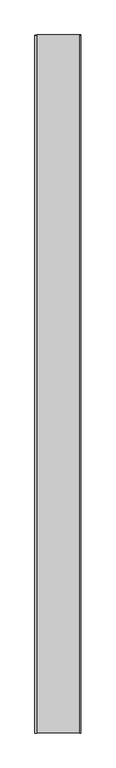
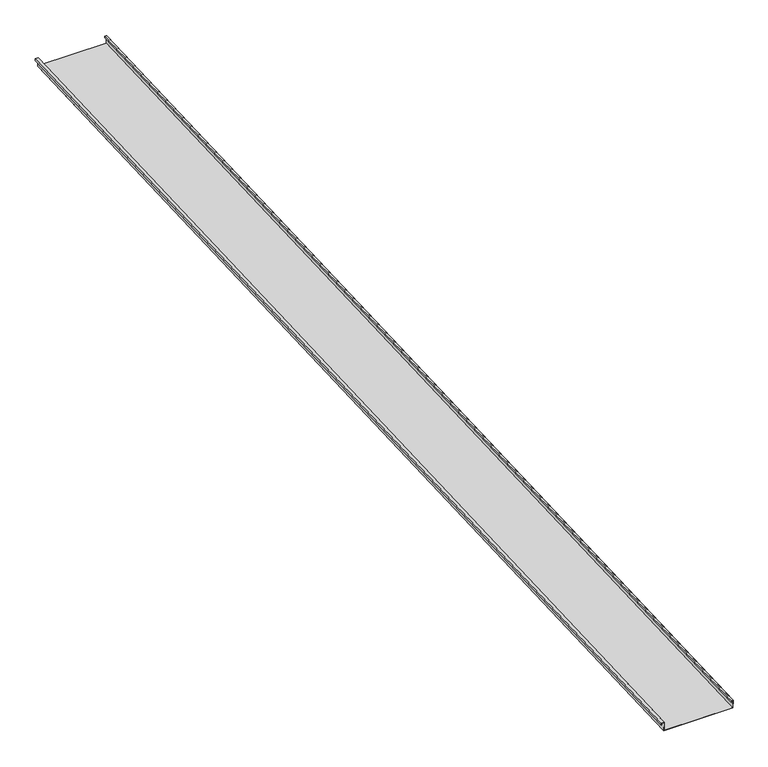
"""IFC4 building model written with IfcOpenShell, lengths in millimetres: proxy geometry, Generic Models 2:Generic Models 2:310765:Generic Models 2:310765 : Generic Models 2:Generic Models 2:310765:99 : Generic Models 2:Generic Models 2:310765:Generic Models 2:310765 : Generic Models 2:Generic Models 2:310765:300385."""

from ifc_helpers import new_model, si_unit, frame, origin, place, context, project, spatial, polyline, outline, extrude, source, transform, mapped, element, save


def generic_models_8109dae2(model_context):
    return source(origin(), model_context, "Body", "SweptSolid", [
        extrude(outline(polyline([(1.5875, 0.0), (1.5875, 50.8), (407.9875, 50.8), (407.9875, 1.5875), (396.875, 1.5875), (396.875, 11.1125), (398.4625, 11.1125), (398.4625, 3.175), (406.4, 3.175), (406.4, 49.2125), (3.175, 49.2125), (3.175, -1.5874999), (-14.2875, -1.5874999), (-14.2875, 9.525), (-12.7, 9.525), (-12.7, 0.0), (1.5875, 0.0)])), frame((614370.5596406, -581354.4345603, 3902.6697972), z_axis=(0.0, 0.9991330730923568, 0.041630544712067834), x_axis=(1.0, 0.0, 0.0)), (0.0, 0.0, 1.0), 6400.8),
    ])


if __name__ == "__main__":
    model = new_model("IFC4")
    model_context = context("Model", 3, world=origin())
    ifc_project = project(units=[si_unit("LENGTHUNIT", "METRE", prefix="MILLI")], contexts=[model_context])
    site = spatial("IfcSite", under=ifc_project)
    building = spatial("IfcBuilding", under=site)
    placement = place(None, origin())
    generic_models_shape = generic_models_8109dae2(model_context)
    element("IfcBuildingElementProxy", 1, Name="Generic Models 2:Generic Models 2:310765:Generic Models 2:310765 : Generic Models 2:Generic Models 2:310765:99 : Generic Models 2:Generic Models 2:310765:Generic Models 2:310765 : Generic Models 2:Generic Models 2:310765:300385", ObjectType="Generic Models 2:Generic Models 2:310765:Generic Models 2:310765 : Generic Models 2:Generic Models 2:310765:99 : Generic Models 2:Generic Models 2:310765:Generic Models 2:310765 : Generic Models 2:Generic Models 2:310765:300385", at=placement, inside=building, context=model_context, shape_type="MappedRepresentation", body=[
        mapped(generic_models_shape, transform((0.0, 0.0, 0.0), x_axis=(1.0, 0.0, 0.0), y_axis=(0.0, 1.0, 0.0), z_axis=(0.0, 0.0, 1.0))),
    ])
    save(model, "model.ifc")

# Revit data of these elements
# Type "Generic Models 2:Generic Models 2:310765:Generic Models 2:310765 : Generic Models 2:Generic Models 2:310765:99 : Generic Models 2:Generic Models 2:310765:Generic Models 2:310765 : Generic Models 2:Generic Models 2:310765:300385"
#   NameOverride = "Generic Models 2:Generic Models 2:310765:Generic Models 2:310765 : Generic Models 2:Generic Models 2:310765:300385"
#   ObjectTypeOverride = "Generic Models 2:310765 : Generic Models 2:Generic Models 2:310765"
#   Reference = "Generic Models 2"
#   Tag = "300385"
# Element 1 (IfcBuildingElementProxy, "Generic Models 2:Generic Models 2:310765:Generic Models 2:310765 : Generic Models 2:Generic Models 2:310765:99 : Generic Models 2:Generic Models 2:310765:Generic Models 2:310765 : Generic Models 2:Generic Models 2:310765:300385")
#   Materials on its faces: "THERMAL BROKEN ALUMINUM STOREFRONT FOR POLYCARBONATE"
# Materials
#   "THERMAL BROKEN ALUMINUM STOREFRONT FOR POLYCARBONATE": class "Unassigned", colour RGB 244 244 244, transparency 0, Keynote = "M07611300.01", Cost = 0
